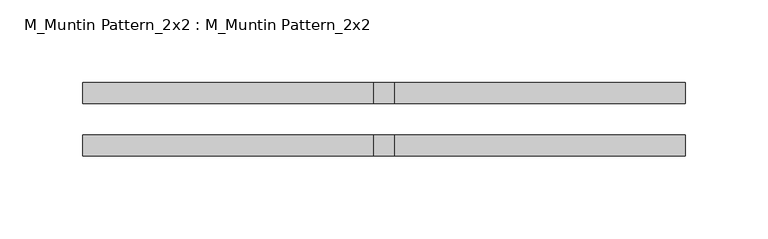
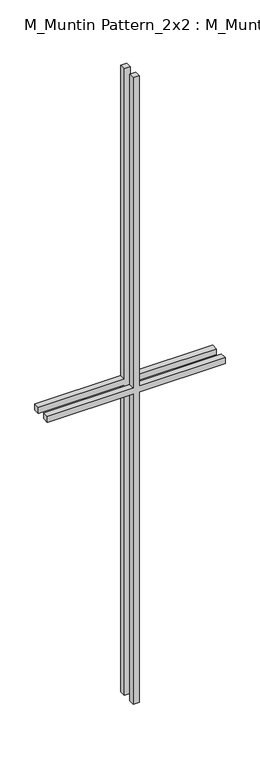
"""IFC4 building model written with IfcOpenShell, lengths in millimetres: proxy geometry, M_Muntin Pattern_2x2 : M_Muntin Pattern_2x2."""

import ifcopenshell
import ifcopenshell.guid

model = None  # the IFC model being written
_history = None  # IfcOwnerHistory: only IFC2X3 demands one
_inside = {}  # id of a spatial element -> (the spatial element, [elements in it])
_under = {}  # id of a project, library or spatial element -> (it, [spatial elements below it])
_declared = {}  # id of a project -> (the project, [libraries it declares])
_typed = {}  # id of a type object -> (the type object, [elements of that type])
_made_of = {}  # id of a material, layer set ... -> (it, [elements and type objects made of it])


def new_model(schema):
    """Start an empty IFC model of exactly this schema.

    Asked for "IFC4X3", IfcOpenShell would pick the latest addendum, in which some entities
    have other attributes; the version numbers below select the first issue.
    IFC2X3 requires an IfcOwnerHistory on every rooted entity: one is made here for all.
    """
    global model, _history
    if schema == "IFC4X3":
        model = ifcopenshell.file(schema_version=(4, 3, 0, 0))
    else:
        model = ifcopenshell.file(schema=schema)
    _inside.clear()
    _under.clear()
    _declared.clear()
    _typed.clear()
    _made_of.clear()
    _history = None
    if model.schema == "IFC2X3":
        org = make("IfcOrganization", Name="unknown")
        user = make(
            "IfcPersonAndOrganization",
            ThePerson=make("IfcPerson", FamilyName="unknown"),
            TheOrganization=org,
        )
        app = make(
            "IfcApplication",
            ApplicationDeveloper=org,
            Version="unknown",
            ApplicationFullName="unknown",
            ApplicationIdentifier="unknown",
        )
        _history = make(
            "IfcOwnerHistory",
            OwningUser=user,
            OwningApplication=app,
            ChangeAction="ADDED",
            CreationDate=0,
        )
    return model


def make(cls, **values):
    """One entity of the class cls with the attributes given. An attribute that is None is left unset."""
    return model.create_entity(
        cls, **{name: value for name, value in values.items() if value is not None}
    )


def rooted(cls, **values):
    """An entity with a GlobalId (a new one), such as an element, a storey or a relation."""
    return make(cls, GlobalId=ifcopenshell.guid.new(), OwnerHistory=_history, **values)


def si_unit(unit_type, name, prefix=None):
    """IfcSIUnit, for example si_unit("LENGTHUNIT", "METRE", prefix="MILLI")."""
    return make("IfcSIUnit", UnitType=unit_type, Prefix=prefix, Name=name)


def assignment(units):
    """IfcUnitAssignment: the units of a project."""
    return None if units is None else make("IfcUnitAssignment", Units=units)


def point(xyz):
    """IfcCartesianPoint."""
    return None if xyz is None else make("IfcCartesianPoint", Coordinates=xyz)


def direction(xyz):
    """IfcDirection."""
    return None if xyz is None else make("IfcDirection", DirectionRatios=xyz)


def frame(location, z_axis=None, x_axis=None):
    """IfcAxis2Placement3D, a coordinate frame: its origin and axes. An axis left out is left unset."""
    return make(
        "IfcAxis2Placement3D",
        Location=point(location),
        Axis=direction(z_axis),
        RefDirection=direction(x_axis),
    )


def origin():
    """The frame at (0, 0, 0) with its axes left unset."""
    return frame((0.0, 0.0, 0.0))


def place(relative_to, where):
    """IfcLocalPlacement: puts the frame where relative to a parent placement (None: the world)."""
    return make(
        "IfcLocalPlacement", PlacementRelTo=relative_to, RelativePlacement=where
    )


def context(
    kind, dimensions, precision=None, world=None, true_north=None, identifier=None
):
    """IfcGeometricRepresentationContext, for example the 3D "Model" context."""
    return make(
        "IfcGeometricRepresentationContext",
        ContextIdentifier=identifier,
        ContextType=kind,
        CoordinateSpaceDimension=dimensions,
        Precision=precision,
        WorldCoordinateSystem=world,
        TrueNorth=true_north,
    )


def project(units=None, contexts=None):
    """IfcProject with its units and contexts."""
    return rooted(
        "IfcProject",
        Name="project",
        RepresentationContexts=contexts,
        UnitsInContext=assignment(units),
    )


def spatial(cls, under=None, at=None, **own):
    """A site, building, storey or space (cls), placed at a placement, below another one or the project."""
    s = rooted(cls, ObjectPlacement=at, **own)
    if under is not None:
        _under.setdefault(under.id(), (under, []))[1].append(s)
    return s


def polyline(points):
    """IfcPolyline through the points."""
    return make("IfcPolyline", Points=[point(p) for p in points])


def outline(outer, holes=None, kind="AREA"):
    """IfcArbitraryClosedProfileDef: a profile drawn as a closed curve; with holes, ...WithVoids."""
    if holes is None:
        return make("IfcArbitraryClosedProfileDef", ProfileType=kind, OuterCurve=outer)
    return make(
        "IfcArbitraryProfileDefWithVoids",
        ProfileType=kind,
        OuterCurve=outer,
        InnerCurves=holes,
    )


def extrude(swept, where, along, depth):
    """IfcExtrudedAreaSolid: the profile swept, set in the frame where, extruded along a direction by depth."""
    return make(
        "IfcExtrudedAreaSolid",
        SweptArea=swept,
        Position=where,
        ExtrudedDirection=direction(along),
        Depth=depth,
    )


def shape(context_of_items, identifier, shape_type, items):
    """IfcShapeRepresentation: the items that make up one representation, for example the "Body"."""
    return make(
        "IfcShapeRepresentation",
        ContextOfItems=context_of_items,
        RepresentationIdentifier=identifier,
        RepresentationType=shape_type,
        Items=items,
    )


def source(mapping_origin, context_of_items, identifier, shape_type, items):
    """IfcRepresentationMap: a shape defined once, which mapped items show again and again."""
    return make(
        "IfcRepresentationMap",
        MappingOrigin=mapping_origin,
        MappedRepresentation=shape(context_of_items, identifier, shape_type, items),
    )


def transform(
    local_origin,
    x_axis=None,
    y_axis=None,
    z_axis=None,
    scale=None,
    scale2=None,
    scale3=None,
    uniform=True,
):
    """IfcCartesianTransformationOperator3D, or its non-uniform kind. x_axis, y_axis, z_axis: its Axis1, 2, 3."""
    if uniform:
        return make(
            "IfcCartesianTransformationOperator3D",
            Axis1=direction(x_axis),
            Axis2=direction(y_axis),
            LocalOrigin=point(local_origin),
            Scale=scale,
            Axis3=direction(z_axis),
        )
    return make(
        "IfcCartesianTransformationOperator3DnonUniform",
        Axis1=direction(x_axis),
        Axis2=direction(y_axis),
        LocalOrigin=point(local_origin),
        Scale=scale,
        Axis3=direction(z_axis),
        Scale2=scale2,
        Scale3=scale3,
    )


def mapped(mapping_source, mapping_target):
    """IfcMappedItem: shows the shape of a source again, moved by a transform."""
    return make(
        "IfcMappedItem", MappingSource=mapping_source, MappingTarget=mapping_target
    )


def made_of(thing, what):
    """Note that an element or type object is made of a material, layer set ...; save() writes the relation."""
    if what is not None:
        _made_of.setdefault(what.id(), (what, []))[1].append(thing)
    return thing


def element(
    cls,
    number,
    at=None,
    inside=None,
    cuts=None,
    type_object=None,
    material=None,
    context=None,
    identifier="Body",
    shape_type=None,
    held_by="IfcProductDefinitionShape",
    body=None,
    shapes=None,
    **own,
):
    """One element of the class cls, such as IfcWall. Its Tag is "e" and its number.

    at: its placement. inside: the storey or other place that contains it. cuts: it is an
    opening in that element (IfcRelVoidsElement). A single representation is given by context,
    identifier, shape_type and body (its items); several are given by shapes. held_by: the class
    of the entity that holds the representations. save() writes the other relations.
    """
    e = rooted(cls, Tag="e%d" % number, ObjectPlacement=at, **own)
    if body is not None:
        shapes = [shape(context, identifier, shape_type, body)]
    if shapes is not None:
        e.Representation = make(held_by, Representations=shapes)
    if inside is not None:
        _inside.setdefault(inside.id(), (inside, []))[1].append(e)
    if cuts is not None:
        rooted(
            "IfcRelVoidsElement", RelatingBuildingElement=cuts, RelatedOpeningElement=e
        )
    if type_object is not None:
        _typed.setdefault(type_object.id(), (type_object, []))[1].append(e)
    return made_of(e, material)


def aggregate(whole, parts):
    """IfcRelAggregates: a whole, such as a stair, and the parts it consists of."""
    return rooted("IfcRelAggregates", RelatingObject=whole, RelatedObjects=parts)


def save(model, path):
    """Write the relations noted so far, then the file.

    IfcRelAggregates (storeys below a building ...), IfcRelContainedInSpatialStructure (elements
    in a storey), IfcRelDefinesByType, IfcRelAssociatesMaterial and IfcRelDeclares: one each for
    every whole, place, type object, material and project.
    """
    for whole, parts in _under.values():
        aggregate(whole, parts)
    for where, things in _inside.values():
        rooted(
            "IfcRelContainedInSpatialStructure",
            RelatedElements=things,
            RelatingStructure=where,
        )
    for kind, things in _typed.values():
        rooted("IfcRelDefinesByType", RelatedObjects=things, RelatingType=kind)
    for what, things in _made_of.values():
        rooted("IfcRelAssociatesMaterial", RelatedObjects=things, RelatingMaterial=what)
    for by, libraries in _declared.values():
        rooted("IfcRelDeclares", RelatingContext=by, RelatedDefinitions=libraries)
    model.write(path)


def m_muntin_pattern_2x2_m_muntin_pattern_2x2_5b5b33da(model_context):
    return source(origin(), model_context, "Body", "SweptSolid", [
        extrude(outline(polyline([(686.5, -6.35), (686.5, -182.2666667), (673.8, -182.2666667), (673.8, -6.35), (0.0, -6.35), (0.0, 6.35), (673.8, 6.35), (673.8, 182.2666667), (686.5, 182.2666667), (686.5, 6.35), (1360.3, 6.35), (1360.3, -6.35), (686.5, -6.35)])), frame((0.0, -22.225, 0.0), z_axis=(0.0, 1.0, 0.0), x_axis=(0.0, 0.0, 1.0)), (0.0, 0.0, 1.0), 12.7),
        extrude(outline(polyline([(686.5, -6.35), (686.5, -182.2666667), (673.8, -182.2666667), (673.8, -6.35), (0.0, -6.35), (0.0, 6.35), (673.8, 6.35), (673.8, 182.2666667), (686.5, 182.2666667), (686.5, 6.35), (1360.3, 6.35), (1360.3, -6.35), (686.5, -6.35)])), frame((0.0, 9.525, 0.0), z_axis=(0.0, 1.0, 0.0), x_axis=(0.0, 0.0, 1.0)), (0.0, 0.0, 1.0), 12.7),
    ])


if __name__ == "__main__":
    model = new_model("IFC4")
    model_context = context("Model", 3, world=origin())
    ifc_project = project(units=[si_unit("LENGTHUNIT", "METRE", prefix="MILLI")], contexts=[model_context])
    site = spatial("IfcSite", under=ifc_project)
    building = spatial("IfcBuilding", under=site)
    placement = place(None, origin())
    m_muntin_pattern_2x2_m_muntin_pattern_2x2_shape = m_muntin_pattern_2x2_m_muntin_pattern_2x2_5b5b33da(model_context)
    element("IfcBuildingElementProxy", 1, Name="M_Muntin Pattern_2x2 : M_Muntin Pattern_2x2", ObjectType="M_Muntin Pattern_2x2 : M_Muntin Pattern_2x2", at=placement, inside=building, context=model_context, shape_type="MappedRepresentation", body=[
        mapped(m_muntin_pattern_2x2_m_muntin_pattern_2x2_shape, transform((0.0, 0.0, 0.0), x_axis=(1.0, 0.0, 0.0), y_axis=(0.0, 1.0, 0.0), z_axis=(0.0, 0.0, 1.0))),
    ])
    save(model, "model.ifc")

# Revit data of these elements
# Type "M_Muntin Pattern_2x2 : M_Muntin Pattern_2x2"
#   Width [instance default] = 1.2 m
#   Thickness = 0.0127 m
#   Height [instance default] = 1.2 m
#   Distance = 0.01905 m
#   Interior Material [instance default] = none
#   Exterior Material [instance default] = none
# Element 1 (IfcBuildingElementProxy, "M_Muntin Pattern_2x2 : M_Muntin Pattern_2x2")
#   Width = 0.364533 m
#   Height = 1.3603 m
#   Interior Material = Wood - Stained
#   Exterior Material = Clad - White
#   Materials on its faces: "Clad - White", "Wood - Stained"
# Materials
#   "Clad - White": class "Wood", colour RGB 242 242 238, transparency 0, Cost = 0
#   "Wood - Stained": class "Wood", colour RGB 224 178 126, transparency 0, Cost = 0
